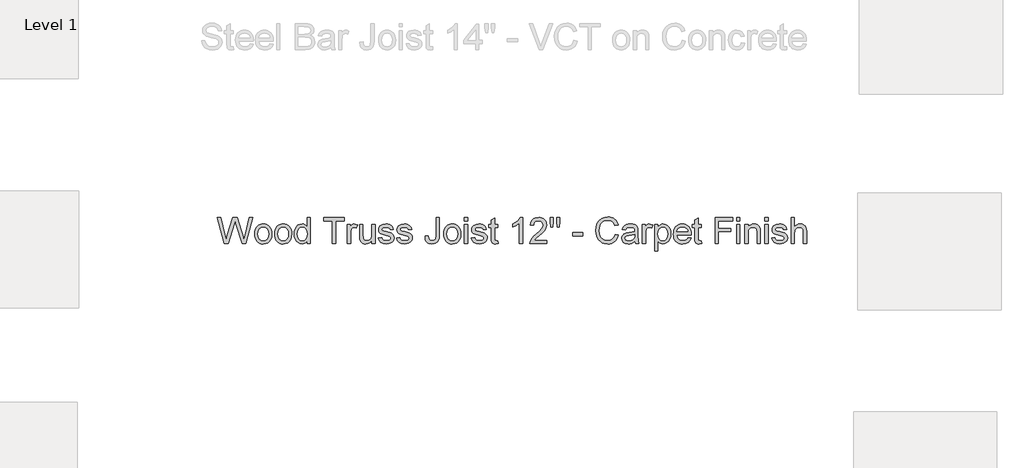
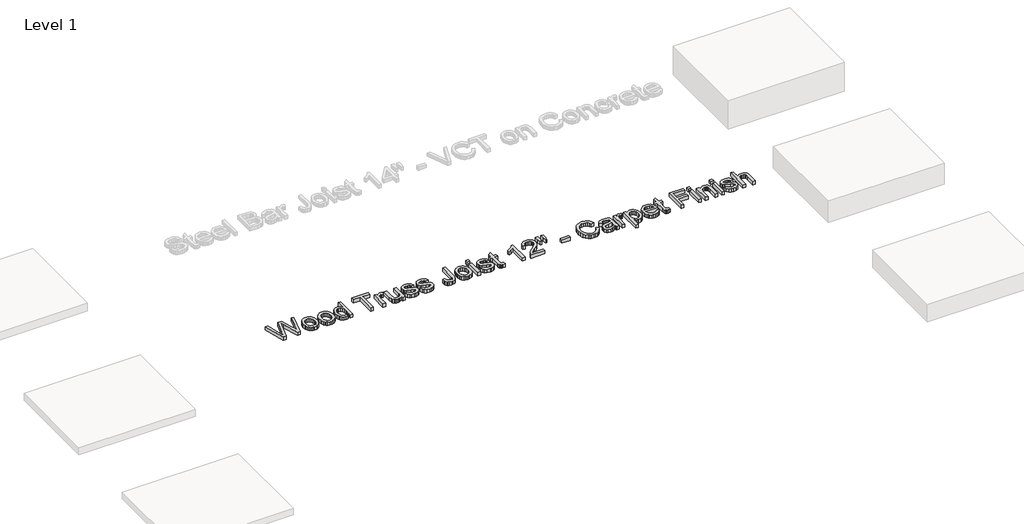
# One storey, part 16 of 42: 1 proxy.
"""IFC4 building model written with IfcOpenShell, lengths in millimetres."""

from ifc_helpers import new_model, si_unit, origin, origin_with_axes, place, context, project, spatial, polyline, outline, extrude, element, save

model = new_model("IFC4")

# Units and contexts
model_context = context("Model", 3, world=origin())
ifc_project = project(units=[si_unit("LENGTHUNIT", "METRE", prefix="MILLI")], contexts=[model_context])

# Site, building, storey
site = spatial("IfcSite", under=ifc_project)
building = spatial("IfcBuilding", under=site)
storey = spatial("IfcBuildingStorey", under=building, Name="Level 1", Elevation=0.0)

# Proxy
placement = place(None, origin())
element("IfcBuildingElementProxy", 1, Name="8\" Arial", ObjectType="8\" Arial", at=placement, inside=storey, context=model_context, shape_type="SweptSolid", body=[
    extrude(outline(polyline([(27173.3571232, -8554.4769735), (27090.30013, -8249.9098794), (27129.5607319, -8249.9098794), (27177.744198, -8450.0794637), (27192.6156381, -8511.8702975), (27208.5280791, -8457.2177549), (27268.9061261, -8249.9098794), (27325.4919558, -8249.9098794), (27369.3627042, -8400.185782), (27388.1564867, -8455.9536825), (27402.0055153, -8511.8702975), (27416.4308122, -8451.8640365), (27465.0604215, -8249.9098794), (27504.3210235, -8249.9098794), (27421.1896731, -8554.4769735), (27380.5162843, -8554.4769735), (27307.4975132, -8319.5082192), (27297.3105767, -8286.7166937), (27285.8595678, -8326.2003673), (27219.3098732, -8554.4769735), (27173.3571232, -8554.4769735)])), origin_with_axes(), (0.0, 0.0, 1.0), 50.8),
    extrude(outline(polyline([(27528.1153277, -8442.6437436), (27530.1740927, -8413.6769666), (27536.3503877, -8388.7161838), (27546.6442126, -8367.7613952), (27561.0555676, -8350.8126007), (27575.5645164, -8339.9796861), (27591.5791985, -8332.2418899), (27609.0996139, -8327.5992122), (27628.1257626, -8326.0516529), (27649.1293482, -8327.9361432), (27668.120642, -8333.5896141), (27685.099644, -8343.0120657), (27700.0663543, -8356.2034978), (27712.2818482, -8372.7177673), (27721.007201, -8392.1087311), (27726.2424126, -8414.376389), (27727.9874832, -8439.5207412), (27724.9016594, -8477.9820032), (27715.6441879, -8507.260151), (27700.4846136, -8529.1862306), (27679.6924813, -8545.591288), (27654.996596, -8555.8246977), (27628.1257626, -8559.2358343), (27606.8154537, -8557.358315), (27587.6475615, -8551.725757), (27570.6220862, -8542.3381604), (27555.7390278, -8529.1955252), (27543.653659, -8512.520923), (27535.0212527, -8492.5374253), (27529.841809, -8469.2450322), (27528.1153277, -8442.6437436)]), holes=[polyline([(27566.1862145, -8442.5693864), (27570.5918786, -8477.0246543), (27583.808871, -8501.5718252), (27603.6994222, -8516.266667), (27628.1257626, -8521.1649475), (27652.4405673, -8516.238783), (27672.2939399, -8501.4602894), (27685.5109323, -8476.5878057), (27689.9165964, -8441.3796712), (27685.4830483, -8407.9282255), (27672.1824041, -8383.7156621), (27652.3011475, -8369.0208203), (27628.1257626, -8364.1225397), (27603.6994222, -8369.002231), (27583.808871, -8383.6413049), (27570.5918786, -8408.1327078), (27566.1862145, -8442.5693864)])]), origin_with_axes(), (0.0, 0.0, 1.0), 50.8),
    extrude(outline(polyline([(27761.2995091, -8442.6437436), (27763.3582741, -8413.6769666), (27769.5345691, -8388.7161838), (27779.828394, -8367.7613952), (27794.239749, -8350.8126007), (27808.7486978, -8339.9796861), (27824.7633799, -8332.2418899), (27842.2837953, -8327.5992122), (27861.309944, -8326.0516529), (27882.3135296, -8327.9361432), (27901.3048234, -8333.5896141), (27918.2838254, -8343.0120657), (27933.2505357, -8356.2034978), (27945.4660296, -8372.7177673), (27954.1913824, -8392.1087311), (27959.426594, -8414.376389), (27961.1716646, -8439.5207412), (27958.0858407, -8477.9820032), (27948.8283693, -8507.260151), (27933.668795, -8529.1862306), (27912.8766627, -8545.591288), (27888.1807774, -8555.8246977), (27861.309944, -8559.2358343), (27839.999635, -8557.358315), (27820.8317429, -8551.725757), (27803.8062676, -8542.3381604), (27788.9232092, -8529.1955252), (27776.8378404, -8512.520923), (27768.2054341, -8492.5374253), (27763.0259903, -8469.2450322), (27761.2995091, -8442.6437436)]), holes=[polyline([(27799.3703959, -8442.5693864), (27803.77606, -8477.0246543), (27816.9930524, -8501.5718252), (27836.8836036, -8516.266667), (27861.309944, -8521.1649475), (27885.6247487, -8516.238783), (27905.4781213, -8501.4602894), (27918.6951137, -8476.5878057), (27923.1007778, -8441.3796712), (27918.6672297, -8407.9282255), (27905.3665855, -8383.7156621), (27885.4853289, -8369.0208203), (27861.309944, -8364.1225397), (27836.8836036, -8369.002231), (27816.9930524, -8383.6413049), (27803.77606, -8408.1327078), (27799.3703959, -8442.5693864)])]), origin_with_axes(), (0.0, 0.0, 1.0), 50.8),
    extrude(outline(polyline([(28142.0083767, -8554.4769735), (28142.0083767, -8518.5624455), (28130.617783, -8536.3570531), (28116.8198749, -8549.0674871), (28100.6146525, -8556.6937475), (28082.0021157, -8559.2358343), (28057.3898823, -8555.5551529), (28034.8596505, -8544.5131086), (28015.7870285, -8526.8811574), (28001.5476246, -8503.4307552), (27992.6805284, -8475.1099564), (27989.7248296, -8442.8668152), (27992.4481621, -8411.023344), (28000.6181595, -8382.2656966), (28014.2255273, -8358.2297315), (28033.2609707, -8340.551307), (28056.2838189, -8329.6765664), (28081.8534013, -8326.0516529), (28100.4798801, -8328.6448603), (28116.95, -8336.4244824), (28130.9105645, -8348.3495185), (28142.0083767, -8363.3789677), (28142.0083767, -8249.9098794), (28180.0792634, -8249.9098794), (28180.0792634, -8554.4769735), (28142.0083767, -8554.4769735)]), holes=[polyline([(28027.7957164, -8442.7181008), (28032.0898447, -8477.1547794), (28044.9722298, -8501.6461824), (28063.691655, -8516.2852563), (28085.4969041, -8521.1649475), (28107.2928586, -8516.5083279), (28125.5382567, -8502.5384688), (28137.8908467, -8478.9951201), (28142.0083767, -8445.6180316), (28137.8164895, -8409.1272354), (28125.2408279, -8383.8271979), (28106.5306973, -8369.0487042), (28083.9354029, -8364.1225397), (28061.9070822, -8368.8535166), (28043.8568718, -8383.0464472), (28031.8110052, -8407.4263144), (28027.7957164, -8442.7181008)])]), origin_with_axes(), (0.0, 0.0, 1.0), 50.8),
    extrude(outline(polyline([(28437.0577491, -8554.4769735), (28437.0577491, -8287.9807662), (28337.1216713, -8287.9807662), (28337.1216713, -8249.9098794), (28575.0647136, -8249.9098794), (28575.0647136, -8287.9807662), (28475.1286358, -8287.9807662), (28475.1286358, -8554.4769735), (28437.0577491, -8554.4769735)])), origin_with_axes(), (0.0, 0.0, 1.0), 50.8),
    extrude(outline(polyline([(28613.1356003, -8554.4769735), (28613.1356003, -8330.8105138), (28646.4476262, -8330.8105138), (28646.4476262, -8363.8994681), (28658.7537429, -8344.7153103), (28670.0932161, -8333.4130158), (28681.4698678, -8327.8919936), (28693.8875203, -8326.0516529), (28712.8486065, -8328.9887623), (28732.1071214, -8337.8000906), (28719.3920401, -8371.9300457), (28706.007744, -8366.0744162), (28692.6234479, -8364.1225397), (28681.2560908, -8366.000059), (28671.0970383, -8371.6326169), (28662.8898622, -8380.5926596), (28657.3781347, -8392.4526331), (28652.749399, -8413.7187925), (28651.2064871, -8436.9182392), (28651.2064871, -8554.4769735), (28613.1356003, -8554.4769735)])), origin_with_axes(), (0.0, 0.0, 1.0), 50.8),
    extrude(outline(polyline([(28898.667251, -8554.4769735), (28898.667251, -8516.0343007), (28884.8925796, -8534.9349717), (28868.8500135, -8548.4354509), (28850.5395529, -8556.5357385), (28829.9611976, -8559.2358343), (28811.4183706, -8557.3397257), (28794.1582054, -8551.6513998), (28779.6771406, -8543.1003218), (28769.4716148, -8532.6159565), (28762.6028684, -8519.8822858), (28758.1321417, -8504.5832918), (28755.9014257, -8469.1892643), (28755.9014257, -8330.8105138), (28793.9723124, -8330.8105138), (28793.9723124, -8451.2691789), (28796.2773856, -8490.0836377), (28801.8262917, -8503.0310852), (28811.3347188, -8512.8741197), (28824.1706306, -8519.0922406), (28839.7019909, -8521.1649475), (28856.1256376, -8519.0457673), (28871.4896941, -8512.6882267), (28884.1583022, -8502.6778885), (28892.4956033, -8489.6003159), (28897.1243391, -8471.6895251), (28898.667251, -8447.1795329), (28898.667251, -8330.8105138), (28936.7381378, -8330.8105138), (28936.7381378, -8554.4769735), (28898.667251, -8554.4769735)])), origin_with_axes(), (0.0, 0.0, 1.0), 50.8),
    extrude(outline(polyline([(28974.8090245, -8487.8529216), (29012.8799113, -8483.0940608), (29018.8842552, -8499.3782877), (29030.5025678, -8511.3497971), (29047.8092063, -8518.7111599), (29070.8785278, -8521.1649475), (29093.6690098, -8518.9156422), (29109.6929866, -8512.1677263), (29119.1735297, -8502.3897544), (29122.3337107, -8491.0502813), (29119.1549404, -8481.3466666), (29109.6186294, -8473.9481251), (29070.4323846, -8463.0919738), (29013.1029829, -8444.465495), (28998.5940341, -8435.1057824), (28988.0817848, -8422.7160138), (28981.6963602, -8408.0862346), (28979.5678854, -8392.0064899), (28981.278101, -8377.2558802), (28986.4087478, -8363.6392179), (28994.4950934, -8351.6955925), (29005.0724052, -8341.9640939), (29029.275674, -8330.698978), (29062.0300209, -8326.0516529), (29086.8095581, -8327.9198776), (29108.354557, -8333.5245516), (29125.6797847, -8342.3172906), (29137.8000085, -8353.7497102), (29145.8305861, -8368.6676236), (29150.8868758, -8387.9168439), (29112.815989, -8392.6757047), (29108.0106549, -8380.6949008), (29098.5022279, -8371.6697955), (29084.1977614, -8366.0093536), (29065.004309, -8364.1225397), (29043.143292, -8365.9257018), (29028.5692806, -8371.3351881), (29020.3713993, -8379.1426942), (29017.6387721, -8388.1399155), (29022.1745614, -8399.2191384), (29036.3767867, -8407.6215021), (29069.1683122, -8415.726437), (29125.0477485, -8433.6465223), (29139.8076529, -8442.2161897), (29150.9984116, -8453.9460381), (29158.053051, -8468.8732462), (29160.4045975, -8487.0349924), (29157.6440864, -8505.8101856), (29149.3625532, -8523.4700208), (29135.8760159, -8538.6295951), (29117.5004927, -8549.9040056), (29095.3048683, -8556.9028771), (29070.3580274, -8559.2358343), (29031.9711226, -8554.7372237), (29003.9570472, -8541.2413917), (28985.2562112, -8518.8970529), (28974.8090245, -8487.8529216)])), origin_with_axes(), (0.0, 0.0, 1.0), 50.8),
    extrude(outline(polyline([(29188.9577625, -8487.8529216), (29227.0286493, -8483.0940608), (29233.0329933, -8499.3782877), (29244.6513059, -8511.3497971), (29261.9579443, -8518.7111599), (29285.0272658, -8521.1649475), (29307.8177479, -8518.9156422), (29323.8417246, -8512.1677263), (29333.3222677, -8502.3897544), (29336.4824487, -8491.0502813), (29333.3036784, -8481.3466666), (29323.7673674, -8473.9481251), (29284.5811226, -8463.0919738), (29227.2517209, -8444.465495), (29212.7427721, -8435.1057824), (29202.2305229, -8422.7160138), (29195.8450983, -8408.0862346), (29193.7166234, -8392.0064899), (29195.426839, -8377.2558802), (29200.5574858, -8363.6392179), (29208.6438314, -8351.6955925), (29219.2211432, -8341.9640939), (29243.4244121, -8330.698978), (29276.178759, -8326.0516529), (29300.9582961, -8327.9198776), (29322.503295, -8333.5245516), (29339.8285228, -8342.3172906), (29351.9487465, -8353.7497102), (29359.9793242, -8368.6676236), (29365.0356138, -8387.9168439), (29326.964727, -8392.6757047), (29322.1593929, -8380.6949008), (29312.6509659, -8371.6697955), (29298.3464994, -8366.0093536), (29279.153047, -8364.1225397), (29257.29203, -8365.9257018), (29242.7180186, -8371.3351881), (29234.5201373, -8379.1426942), (29231.7875101, -8388.1399155), (29236.3232994, -8399.2191384), (29250.5255247, -8407.6215021), (29283.3170502, -8415.726437), (29339.1964866, -8433.6465223), (29353.9563909, -8442.2161897), (29365.1471496, -8453.9460381), (29372.201789, -8468.8732462), (29374.5533355, -8487.0349924), (29371.7928244, -8505.8101856), (29363.5112912, -8523.4700208), (29350.0247539, -8538.6295951), (29331.6492307, -8549.9040056), (29309.4536063, -8556.9028771), (29284.5067654, -8559.2358343), (29246.1198606, -8554.7372237), (29218.1057852, -8541.2413917), (29199.4049492, -8518.8970529), (29188.9577625, -8487.8529216)])), origin_with_axes(), (0.0, 0.0, 1.0), 50.8),
    extrude(outline(polyline([(29522.0780217, -8468.9661927), (29560.1489084, -8464.0586174), (29564.1084294, -8491.7380854), (29573.1614186, -8509.0447238), (29586.9918579, -8518.1348916), (29605.2837293, -8521.1649475), (29619.3465348, -8519.4454373), (29631.3459281, -8514.2869065), (29640.6033996, -8506.1633823), (29646.4404398, -8495.5488919), (29650.5672645, -8457.8126126), (29650.5672645, -8249.9098794), (29688.6381512, -8249.9098794), (29688.6381512, -8457.1433977), (29686.3423727, -8491.0409866), (29679.455037, -8516.2945509), (29667.5764741, -8534.7444313), (29650.3070143, -8548.2309686), (29628.6225956, -8556.4846179), (29603.4991564, -8559.2358343), (29568.3096112, -8553.5568031), (29554.2142744, -8546.4580141), (29542.4518947, -8536.5197095), (29533.2316018, -8523.7790679), (29526.7625253, -8508.2732679), (29522.0780217, -8468.9661927)])), origin_with_axes(), (0.0, 0.0, 1.0), 50.8),
    extrude(outline(polyline([(29740.9856205, -8442.6437436), (29743.0443855, -8413.6769666), (29749.2206805, -8388.7161838), (29759.5145055, -8367.7613952), (29773.9258604, -8350.8126007), (29788.4348092, -8339.9796861), (29804.4494913, -8332.2418899), (29821.9699068, -8327.5992122), (29840.9960555, -8326.0516529), (29861.999641, -8327.9361432), (29880.9909348, -8333.5896141), (29897.9699369, -8343.0120657), (29912.9366472, -8356.2034978), (29925.152141, -8372.7177673), (29933.8774938, -8392.1087311), (29939.1127055, -8414.376389), (29940.857776, -8439.5207412), (29937.7719522, -8477.9820032), (29928.5144807, -8507.260151), (29913.3549064, -8529.1862306), (29892.5627742, -8545.591288), (29867.8668889, -8555.8246977), (29840.9960555, -8559.2358343), (29819.6857465, -8557.358315), (29800.5178543, -8551.725757), (29783.4923791, -8542.3381604), (29768.6093206, -8529.1955252), (29756.5239518, -8512.520923), (29747.8915456, -8492.5374253), (29742.7121018, -8469.2450322), (29740.9856205, -8442.6437436)]), holes=[polyline([(29779.0565073, -8442.5693864), (29783.4621714, -8477.0246543), (29796.6791639, -8501.5718252), (29816.5697151, -8516.266667), (29840.9960555, -8521.1649475), (29865.3108601, -8516.238783), (29885.1642327, -8501.4602894), (29898.3812251, -8476.5878057), (29902.7868893, -8441.3796712), (29898.3533412, -8407.9282255), (29885.0526969, -8383.7156621), (29865.1714404, -8369.0208203), (29840.9960555, -8364.1225397), (29816.5697151, -8369.002231), (29796.6791639, -8383.6413049), (29783.4621714, -8408.1327078), (29779.0565073, -8442.5693864)])]), origin_with_axes(), (0.0, 0.0, 1.0), 50.8),
    extrude(outline(polyline([(29983.6875236, -8287.9807662), (29983.6875236, -8249.9098794), (30021.7584104, -8249.9098794), (30021.7584104, -8287.9807662), (29983.6875236, -8287.9807662)])), origin_with_axes(), (0.0, 0.0, 1.0), 50.8),
    extrude(outline(polyline([(29983.6875236, -8554.4769735), (29983.6875236, -8330.8105138), (30021.7584104, -8330.8105138), (30021.7584104, -8554.4769735), (29983.6875236, -8554.4769735)])), origin_with_axes(), (0.0, 0.0, 1.0), 50.8),
    extrude(outline(polyline([(30064.588158, -8487.8529216), (30102.6590447, -8483.0940608), (30108.6633887, -8499.3782877), (30120.2817013, -8511.3497971), (30137.5883398, -8518.7111599), (30160.6576613, -8521.1649475), (30183.4481433, -8518.9156422), (30199.4721201, -8512.1677263), (30208.9526631, -8502.3897544), (30212.1128442, -8491.0502813), (30208.9340738, -8481.3466666), (30199.3977629, -8473.9481251), (30160.2115181, -8463.0919738), (30102.8821163, -8444.465495), (30088.3731676, -8435.1057824), (30077.8609183, -8422.7160138), (30071.4754937, -8408.0862346), (30069.3470188, -8392.0064899), (30071.0572344, -8377.2558802), (30076.1878813, -8363.6392179), (30084.2742269, -8351.6955925), (30094.8515387, -8341.9640939), (30119.0548075, -8330.698978), (30151.8091544, -8326.0516529), (30176.5886915, -8327.9198776), (30198.1336904, -8333.5245516), (30215.4589182, -8342.3172906), (30227.5791419, -8353.7497102), (30235.6097196, -8368.6676236), (30240.6660092, -8387.9168439), (30202.5951225, -8392.6757047), (30197.7897884, -8380.6949008), (30188.2813614, -8371.6697955), (30173.9768949, -8366.0093536), (30154.7834424, -8364.1225397), (30132.9224254, -8365.9257018), (30118.3484141, -8371.3351881), (30110.1505327, -8379.1426942), (30107.4179056, -8388.1399155), (30111.9536948, -8399.2191384), (30126.1559202, -8407.6215021), (30158.9474457, -8415.726437), (30214.826882, -8433.6465223), (30229.5867863, -8442.2161897), (30240.777545, -8453.9460381), (30247.8321845, -8468.8732462), (30250.1837309, -8487.0349924), (30247.4232199, -8505.8101856), (30239.1416866, -8523.4700208), (30225.6551494, -8538.6295951), (30207.2796261, -8549.9040056), (30185.0840017, -8556.9028771), (30160.1371609, -8559.2358343), (30121.750256, -8554.7372237), (30093.7361807, -8541.2413917), (30075.0353447, -8518.8970529), (30064.588158, -8487.8529216)])), origin_with_axes(), (0.0, 0.0, 1.0), 50.8),
    extrude(outline(polyline([(30373.9141129, -8522.7264488), (30378.6729737, -8555.5923315), (30350.1941659, -8559.2358343), (30331.9208838, -8557.6557438), (30318.2949268, -8552.9154722), (30308.6656693, -8545.6098773), (30302.3824858, -8536.3338165), (30298.924876, -8520.4027862), (30297.7723394, -8493.1322829), (30297.7723394, -8368.8814005), (30269.2191743, -8368.8814005), (30269.2191743, -8330.8105138), (30297.7723394, -8330.8105138), (30297.7723394, -8276.4554), (30335.8432261, -8254.0738826), (30335.8432261, -8330.8105138), (30373.9141129, -8330.8105138), (30373.9141129, -8368.8814005), (30335.8432261, -8368.8814005), (30335.8432261, -8492.0169249), (30337.8508706, -8511.6472259), (30344.3571256, -8518.5996241), (30357.3324571, -8521.1649475), (30373.9141129, -8522.7264488)])), origin_with_axes(), (0.0, 0.0, 1.0), 50.8),
    extrude(outline(polyline([(30664.2046244, -8554.4769735), (30626.1337377, -8554.4769735), (30626.1337377, -8317.1287888), (30590.0704953, -8342.8192017), (30549.9919642, -8362.040538), (30549.9919642, -8326.0516529), (30579.8928535, -8309.7860153), (30605.7970433, -8290.4345538), (30626.2173895, -8269.8561985), (30639.6667482, -8249.9098794), (30664.2046244, -8249.9098794), (30664.2046244, -8554.4769735)])), origin_with_axes(), (0.0, 0.0, 1.0), 50.8),
    extrude(outline(polyline([(30949.7362751, -8516.4060867), (30949.7362751, -8554.4769735), (30749.8641196, -8554.4769735), (30753.9537657, -8528.2288816), (30763.3413623, -8507.7155889), (30777.0788551, -8487.815743), (30796.950817, -8466.9864322), (30824.7418207, -8443.6847444), (30865.8241741, -8407.1939482), (30890.4735862, -8380.2580522), (30902.7982922, -8358.3970352), (30906.9065275, -8337.1308758), (30903.0306584, -8318.0675485), (30891.4030512, -8302.2201701), (30873.5294391, -8291.5406171), (30850.9155554, -8287.9807662), (30827.1677244, -8291.4569653), (30808.717844, -8301.8855627), (30796.8113972, -8318.4486291), (30792.6938672, -8340.3282354), (30754.6229805, -8335.5693746), (30757.897021, -8315.915837), (30763.852568, -8298.743971), (30772.4896216, -8284.0537765), (30783.8081818, -8271.8452536), (30797.5479983, -8262.2485274), (30813.4488209, -8255.3937229), (30851.7334846, -8249.9098794), (30872.1375652, -8251.434202), (30890.2969878, -8256.0071699), (30906.2117524, -8263.6287829), (30919.881859, -8274.2990412), (30930.8611645, -8287.2278995), (30938.7035255, -8301.6253125), (30943.4089421, -8317.4912802), (30944.9774143, -8334.8258026), (30943.285788, -8353.0340221), (30938.210909, -8370.9262235), (30929.2043931, -8389.1251484), (30915.7178558, -8408.2535383), (30894.2193301, -8431.0904936), (30861.1768491, -8460.4151146), (30817.3804579, -8497.0360359), (30800.2039445, -8516.4060867), (30949.7362751, -8516.4060867)])), origin_with_axes(), (0.0, 0.0, 1.0), 50.8),
    extrude(outline(polyline([(30997.101812, -8359.3636788), (30987.8071619, -8300.5471331), (30987.8071619, -8249.9098794), (31025.8780486, -8249.9098794), (31025.8780486, -8300.5471331), (31017.5500422, -8359.3636788), (30997.101812, -8359.3636788)])), origin_with_axes(), (0.0, 0.0, 1.0), 50.8),
    extrude(outline(polyline([(31073.0205139, -8359.3636788), (31063.9489354, -8300.5471331), (31063.9489354, -8249.9098794), (31102.0198222, -8249.9098794), (31102.0198222, -8300.5471331), (31093.0969581, -8359.3636788), (31073.0205139, -8359.3636788)])), origin_with_axes(), (0.0, 0.0, 1.0), 50.8),
    extrude(outline(polyline([(31249.5445083, -8464.0586174), (31249.5445083, -8425.9877307), (31368.5160295, -8425.9877307), (31368.5160295, -8464.0586174), (31249.5445083, -8464.0586174)])), origin_with_axes(), (0.0, 0.0, 1.0), 50.8),
    extrude(outline(polyline([(31749.2248971, -8446.2128892), (31787.2957838, -8456.0280397), (31779.7624699, -8479.7038372), (31769.7288951, -8500.3914046), (31757.1950595, -8518.090742), (31742.160963, -8532.8018495), (31724.9658603, -8544.3667178), (31705.9490062, -8552.6273381), (31685.1104007, -8557.5837103), (31662.4500438, -8559.2358343), (31618.2911613, -8554.2353126), (31599.6205329, -8547.9846604), (31583.2224465, -8539.2337473), (31556.3423184, -8514.751639), (31536.7491961, -8481.309488), (31524.7869814, -8441.9931181), (31520.7995765, -8399.8883532), (31525.3074818, -8355.4785151), (31538.8311977, -8317.1287888), (31560.6643307, -8286.0567736), (31590.1004876, -8263.4800685), (31625.0111933, -8249.733281), (31663.267973, -8245.1510185), (31685.0430145, -8246.6335152), (31705.0102466, -8251.0810053), (31723.1696692, -8258.4934887), (31739.5212824, -8268.8709656), (31753.7955412, -8281.9392436), (31765.722901, -8297.4241306), (31782.536923, -8335.6437318), (31744.4660362, -8344.7153103), (31731.2676331, -8316.9521905), (31713.2360119, -8297.9074524), (31690.1481011, -8286.8932921), (31661.780829, -8283.2219053), (31629.08225, -8287.292962), (31602.2207113, -8299.5061323), (31581.8375436, -8318.5787542), (31568.5740779, -8343.2281663), (31561.2963669, -8371.0935272), (31558.8704633, -8399.813996), (31561.7425101, -8434.9849519), (31570.3586508, -8465.397047), (31585.0441979, -8489.88845), (31606.1244643, -8507.2973296), (31631.3966179, -8517.6980431), (31658.6578266, -8521.1649475), (31690.4362352, -8516.4432653), (31716.9166933, -8502.2782186), (31736.9094857, -8478.8185217), (31749.2248971, -8446.2128892)])), origin_with_axes(), (0.0, 0.0, 1.0), 50.8),
    extrude(outline(polyline([(31977.6502176, -8525.9238084), (31959.4605874, -8541.5202312), (31940.7318675, -8551.725757), (31921.0365039, -8557.358315), (31899.9469429, -8559.2358343), (31868.1313556, -8554.7186344), (31844.6623641, -8541.1670345), (31830.190594, -8520.5886792), (31825.3666706, -8494.9912129), (31827.188422, -8479.2088971), (31832.6536762, -8464.8765466), (31841.0839239, -8452.6076085), (31851.8006554, -8443.0155296), (31878.4577119, -8430.5235199), (31911.3979518, -8424.7980154), (31950.3239463, -8418.7750822), (31977.427146, -8411.7111481), (31977.6502176, -8403.2344272), (31975.0291263, -8386.2438069), (31967.1658523, -8375.1274054), (31949.5803743, -8366.8737561), (31925.0796767, -8364.1225397), (31902.4007305, -8365.9535857), (31886.5626467, -8371.4467239), (31875.7622633, -8381.6057765), (31868.1964182, -8397.4345656), (31830.1255314, -8392.6757047), (31836.7340276, -8371.8556885), (31846.5956514, -8355.4971044), (31860.630573, -8342.9865054), (31879.7589629, -8333.7104446), (31903.1535972, -8327.9663508), (31929.987252, -8326.0516529), (31955.724138, -8327.7432792), (31976.125895, -8332.8181582), (31991.5085409, -8340.4490659), (32002.1880938, -8349.8087785), (32009.2706172, -8361.3806179), (32013.8621743, -8375.6479058), (32015.7211044, -8408.9599317), (32015.7211044, -8456.3254685), (32017.6543916, -8522.4661986), (32025.2388261, -8554.4769735), (31987.1679393, -8554.4769735), (31981.0706488, -8541.2413917), (31977.6502176, -8525.9238084)]), holes=[polyline([(31977.6502176, -8449.7820349), (31916.2311698, -8461.4561154), (31883.4768229, -8467.627763), (31868.6425614, -8477.6659851), (31863.4375573, -8492.3143537), (31866.2724256, -8503.6352375), (31874.7770304, -8512.9112983), (31888.7654788, -8519.1015352), (31908.0518777, -8521.1649475), (31928.5001079, -8518.8877583), (31946.5689077, -8512.0561905), (31961.2172762, -8501.9900844), (31971.4042127, -8490.0092805), (31975.9214127, -8477.6659851), (31977.427146, -8460.563829), (31977.6502176, -8449.7820349)])]), origin_with_axes(), (0.0, 0.0, 1.0), 50.8),
    extrude(outline(polyline([(32068.0685737, -8554.4769735), (32068.0685737, -8330.8105138), (32101.3805996, -8330.8105138), (32101.3805996, -8363.8994681), (32113.6867163, -8344.7153103), (32125.0261894, -8333.4130158), (32136.4028411, -8327.8919936), (32148.8204936, -8326.0516529), (32167.7815798, -8328.9887623), (32187.0400948, -8337.8000906), (32174.3250135, -8371.9300457), (32160.9407173, -8366.0744162), (32147.5564212, -8364.1225397), (32136.1890641, -8366.000059), (32126.0300116, -8371.6326169), (32117.8228356, -8380.5926596), (32112.3111081, -8392.4526331), (32107.6823723, -8413.7187925), (32106.1394604, -8436.9182392), (32106.1394604, -8554.4769735), (32068.0685737, -8554.4769735)])), origin_with_axes(), (0.0, 0.0, 1.0), 50.8),
    extrude(outline(polyline([(32210.834399, -8640.1364687), (32210.834399, -8330.8105138), (32248.9052858, -8330.8105138), (32248.9052858, -8368.1378285), (32261.3229383, -8349.7251267), (32275.2277348, -8336.5731968), (32291.4376046, -8328.6820389), (32310.7704767, -8326.0516529), (32336.5166575, -8329.7323343), (32359.0283, -8340.7743786), (32377.35735, -8358.508571), (32390.5557531, -8382.2656966), (32398.5305629, -8410.3169506), (32401.1888328, -8440.933528), (32398.1866608, -8473.4926872), (32389.1801449, -8502.612826), (32374.4574191, -8526.8160948), (32354.3066177, -8544.6246444), (32330.8376263, -8555.5830368), (32306.1603303, -8559.2358343), (32288.6585042, -8556.7913413), (32273.0341974, -8549.4578624), (32259.6591959, -8538.3879342), (32248.9052858, -8524.7340932), (32248.9052858, -8640.1364687), (32210.834399, -8640.1364687)]), holes=[polyline([(32248.9052858, -8444.4283164), (32253.0228157, -8478.5582715), (32265.3754057, -8502.426933), (32283.6022145, -8516.4804439), (32305.3424011, -8521.1649475), (32327.4357843, -8516.3131402), (32346.1273257, -8501.7577182), (32358.8702909, -8477.0153596), (32363.117946, -8441.6027428), (32358.9725321, -8407.6586807), (32346.5362903, -8383.4554119), (32328.3373654, -8368.9557577), (32306.9039023, -8364.1225397), (32285.3867874, -8369.2624812), (32266.4907637, -8384.6823057), (32253.3016552, -8409.8986914), (32248.9052858, -8444.4283164)])]), origin_with_axes(), (0.0, 0.0, 1.0), 50.8),
    extrude(outline(polyline([(32600.6148451, -8487.8529216), (32637.9421598, -8492.6117825), (32624.4928011, -8520.7373936), (32603.0314541, -8541.7618921), (32574.0414405, -8554.8673488), (32538.0060821, -8559.2358343), (32514.3837289, -8557.351344), (32493.3359938, -8551.6978731), (32474.8628767, -8542.2754216), (32458.9643777, -8529.0839894), (32446.1795865, -8512.4907154), (32437.0475928, -8492.862738), (32431.5683966, -8470.2000575), (32429.7419979, -8444.5026736), (32431.5869859, -8417.9339164), (32437.12195, -8394.5160455), (32446.3468902, -8374.2490609), (32459.2618065, -8357.1329628), (32475.1184796, -8343.5348897), (32493.1686901, -8333.8219804), (32513.4124379, -8327.9942348), (32535.8497233, -8326.0516529), (32557.5643495, -8327.9895875), (32577.2016215, -8333.8033911), (32594.7615392, -8343.4930638), (32610.2441026, -8357.0586056), (32622.882503, -8374.1375251), (32631.9099319, -8394.3673311), (32637.3263893, -8417.7480233), (32639.131875, -8444.279602), (32638.9088034, -8454.5408957), (32467.8128846, -8454.5408957), (32474.4027915, -8483.0382929), (32489.7110802, -8503.9884342), (32511.8044635, -8516.8708192), (32538.7496541, -8521.1649475), (32559.0119913, -8519.1758924), (32576.0769688, -8513.2087271), (32589.9445868, -8502.8916655), (32600.6148451, -8487.8529216)]), holes=[polyline([(32467.8128846, -8416.470009), (32601.0609883, -8416.470009), (32595.9117521, -8396.3563862), (32585.8177621, -8381.9682678), (32563.6221377, -8368.5839717), (32535.7010089, -8364.1225397), (32510.03848, -8367.6823907), (32488.8187938, -8378.3619436), (32474.0681841, -8395.0086619), (32467.8128846, -8416.470009)])]), origin_with_axes(), (0.0, 0.0, 1.0), 50.8),
    extrude(outline(polyline([(32758.1033962, -8522.7264488), (32762.862257, -8555.5923315), (32734.3834491, -8559.2358343), (32716.1101671, -8557.6557438), (32702.48421, -8552.9154722), (32692.8549525, -8545.6098773), (32686.5717691, -8536.3338165), (32683.1141592, -8520.4027862), (32681.9616226, -8493.1322829), (32681.9616226, -8368.8814005), (32653.4084576, -8368.8814005), (32653.4084576, -8330.8105138), (32681.9616226, -8330.8105138), (32681.9616226, -8276.4554), (32720.0325094, -8254.0738826), (32720.0325094, -8330.8105138), (32758.1033962, -8330.8105138), (32758.1033962, -8368.8814005), (32720.0325094, -8368.8814005), (32720.0325094, -8492.0169249), (32722.0401538, -8511.6472259), (32728.5464089, -8518.5996241), (32741.5217404, -8521.1649475), (32758.1033962, -8522.7264488)])), origin_with_axes(), (0.0, 0.0, 1.0), 50.8),
    extrude(outline(polyline([(32919.9046649, -8554.4769735), (32919.9046649, -8249.9098794), (33124.5356812, -8249.9098794), (33124.5356812, -8287.9807662), (32957.9755516, -8287.9807662), (32957.9755516, -8378.3991222), (33100.741377, -8378.3991222), (33100.741377, -8416.470009), (32957.9755516, -8416.470009), (32957.9755516, -8554.4769735), (32919.9046649, -8554.4769735)])), origin_with_axes(), (0.0, 0.0, 1.0), 50.8),
    extrude(outline(polyline([(33172.1242897, -8287.9807662), (33172.1242897, -8249.9098794), (33210.1951764, -8249.9098794), (33210.1951764, -8287.9807662), (33172.1242897, -8287.9807662)])), origin_with_axes(), (0.0, 0.0, 1.0), 50.8),
    extrude(outline(polyline([(33172.1242897, -8554.4769735), (33172.1242897, -8330.8105138), (33210.1951764, -8330.8105138), (33210.1951764, -8554.4769735), (33172.1242897, -8554.4769735)])), origin_with_axes(), (0.0, 0.0, 1.0), 50.8),
    extrude(outline(polyline([(33267.3015065, -8554.4769735), (33267.3015065, -8330.8105138), (33305.3723933, -8330.8105138), (33305.3723933, -8362.040538), (33318.5986804, -8346.2954008), (33334.4832374, -8335.0488742), (33353.0260643, -8328.3009582), (33374.2271612, -8326.0516529), (33392.9930597, -8327.8641097), (33410.1788677, -8333.30148), (33424.5112181, -8341.6852544), (33434.7167439, -8352.3369234), (33446.1305742, -8380.3324094), (33448.1382187, -8417.1392238), (33448.1382187, -8554.4769735), (33410.0673319, -8554.4769735), (33410.0673319, -8422.2698706), (33405.6802571, -8388.5860587), (33399.6108505, -8378.5571313), (33390.1767807, -8370.7775091), (33378.0844409, -8365.786282), (33364.0402247, -8364.1225397), (33341.7423591, -8367.858989), (33322.7347997, -8379.068337), (33315.1387469, -8388.21892), (33309.7129949, -8400.7248717), (33305.3723933, -8435.8028811), (33305.3723933, -8554.4769735), (33267.3015065, -8554.4769735)])), origin_with_axes(), (0.0, 0.0, 1.0), 50.8),
    extrude(outline(polyline([(33500.4856879, -8287.9807662), (33500.4856879, -8249.9098794), (33538.5565747, -8249.9098794), (33538.5565747, -8287.9807662), (33500.4856879, -8287.9807662)])), origin_with_axes(), (0.0, 0.0, 1.0), 50.8),
    extrude(outline(polyline([(33500.4856879, -8554.4769735), (33500.4856879, -8330.8105138), (33538.5565747, -8330.8105138), (33538.5565747, -8554.4769735), (33500.4856879, -8554.4769735)])), origin_with_axes(), (0.0, 0.0, 1.0), 50.8),
    extrude(outline(polyline([(33581.3863223, -8487.8529216), (33619.4572091, -8483.0940608), (33625.461553, -8499.3782877), (33637.0798656, -8511.3497971), (33654.3865041, -8518.7111599), (33677.4558256, -8521.1649475), (33700.2463076, -8518.9156422), (33716.2702844, -8512.1677263), (33725.7508275, -8502.3897544), (33728.9110085, -8491.0502813), (33725.7322382, -8481.3466666), (33716.1959272, -8473.9481251), (33677.0096824, -8463.0919738), (33619.6802807, -8444.465495), (33605.1713319, -8435.1057824), (33594.6590826, -8422.7160138), (33588.273658, -8408.0862346), (33586.1451832, -8392.0064899), (33587.8553988, -8377.2558802), (33592.9860456, -8363.6392179), (33601.0723912, -8351.6955925), (33611.649703, -8341.9640939), (33635.8529718, -8330.698978), (33668.6073187, -8326.0516529), (33693.3868559, -8327.9198776), (33714.9318548, -8333.5245516), (33732.2570825, -8342.3172906), (33744.3773062, -8353.7497102), (33752.4078839, -8368.6676236), (33757.4641736, -8387.9168439), (33719.3932868, -8392.6757047), (33714.5879527, -8380.6949008), (33705.0795257, -8371.6697955), (33690.7750592, -8366.0093536), (33671.5816068, -8364.1225397), (33649.7205897, -8365.9257018), (33635.1465784, -8371.3351881), (33626.948697, -8379.1426942), (33624.2160699, -8388.1399155), (33628.7518592, -8399.2191384), (33642.9540845, -8407.6215021), (33675.74561, -8415.726437), (33731.6250463, -8433.6465223), (33746.3849507, -8442.2161897), (33757.5757094, -8453.9460381), (33764.6303488, -8468.8732462), (33766.9818953, -8487.0349924), (33764.2213842, -8505.8101856), (33755.9398509, -8523.4700208), (33742.4533137, -8538.6295951), (33724.0777904, -8549.9040056), (33701.882166, -8556.9028771), (33676.9353252, -8559.2358343), (33638.5484203, -8554.7372237), (33610.534345, -8541.2413917), (33591.833509, -8518.8970529), (33581.3863223, -8487.8529216)])), origin_with_axes(), (0.0, 0.0, 1.0), 50.8),
    extrude(outline(polyline([(33809.8116429, -8554.4769735), (33809.8116429, -8249.9098794), (33847.8825296, -8249.9098794), (33847.8825296, -8361.8918236), (33861.8663307, -8346.211749), (33877.569642, -8335.0116956), (33894.9924636, -8328.2916636), (33914.1347954, -8326.0516529), (33937.1297598, -8328.4961459), (33956.8901858, -8335.8296248), (33972.4494301, -8347.4758214), (33982.8408489, -8362.8584673), (33988.6964784, -8383.9945016), (33990.648355, -8412.9008633), (33990.648355, -8554.4769735), (33952.5774682, -8554.4769735), (33952.5774682, -8416.841795), (33949.5474123, -8393.0103121), (33940.4572445, -8376.6889066), (33925.8088759, -8367.2641314), (33906.1042178, -8364.1225397), (33890.0151785, -8366.2417199), (33874.9113721, -8372.5992605), (33862.4007731, -8382.5817147), (33854.0913559, -8395.5756356), (33849.4347362, -8412.8450954), (33847.8825296, -8435.6541667), (33847.8825296, -8554.4769735), (33809.8116429, -8554.4769735)])), origin_with_axes(), (0.0, 0.0, 1.0), 50.8),
])

save(model, "model.ifc")

# Revit data of these elements
# Element 1 (IfcBuildingElementProxy, "8\" Arial")
#   Phase Created = New Construction
